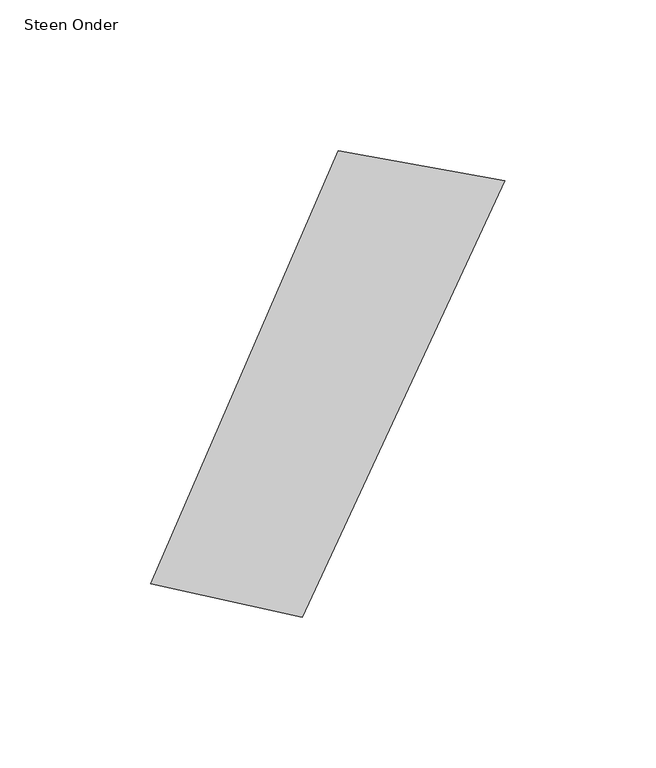
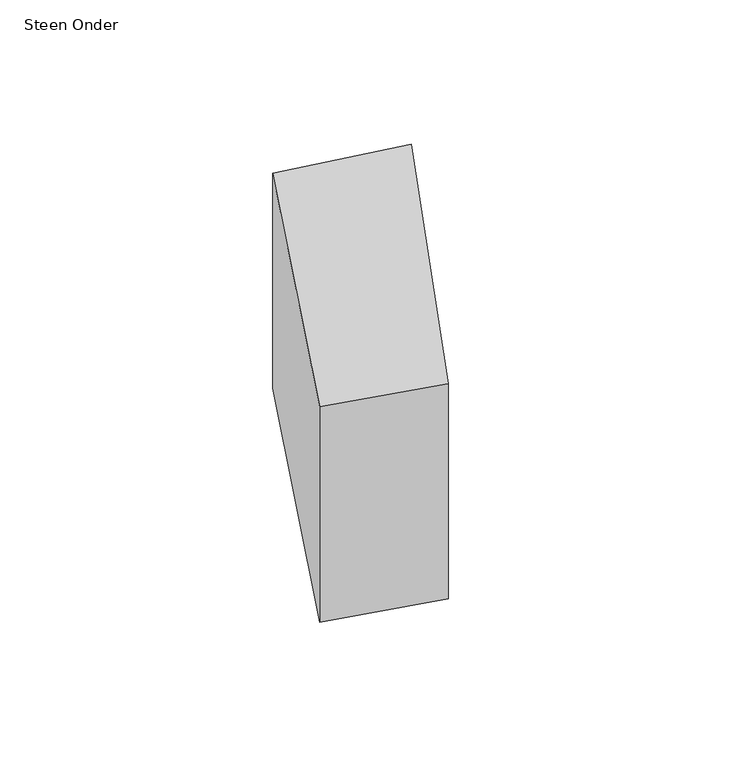
"""IFC4 building model written with IfcOpenShell, lengths in millimetres: proxy geometry, 00_GMA_steen_versie_4 : Steen Onder."""

from ifc_helpers import new_model, si_unit, origin, origin_with_axes, place, context, project, spatial, polyline, outline, extrude, source, transform, mapped, element, save


def steen_onder_ea4eff59(model_context):
    return source(origin(), model_context, "Body", "SweptSolid", [
        extrude(outline(polyline([(133.1834869, 139.6210071), (66.0338965, -4.9121836), (15.9385421, 6.1101542), (77.9749462, 149.4742626), (133.1834869, 139.6210071)])), origin_with_axes(), (0.0, 0.0, 1.0), 100.0),
    ])


if __name__ == "__main__":
    model = new_model("IFC4")
    model_context = context("Model", 3, world=origin())
    ifc_project = project(units=[si_unit("LENGTHUNIT", "METRE", prefix="MILLI")], contexts=[model_context])
    site = spatial("IfcSite", under=ifc_project)
    building = spatial("IfcBuilding", under=site)
    placement = place(None, origin())
    steen_onder_shape = steen_onder_ea4eff59(model_context)
    element("IfcBuildingElementProxy", 1, Name="00_GMA_steen_versie_4 : Steen Onder", ObjectType="00_GMA_steen_versie_4 : Steen Onder", at=placement, inside=building, context=model_context, shape_type="MappedRepresentation", body=[
        mapped(steen_onder_shape, transform((0.0, 0.0, 0.0), x_axis=(1.0, 0.0, 0.0), y_axis=(0.0, 1.0, 0.0), z_axis=(0.0, 0.0, 1.0))),
    ])
    save(model, "model.ifc")

# Revit data of these elements
# Type "00_GMA_steen_versie_4 : Steen Onder"
#   StootVoegHalfBoven [instance default] = 5 mm
#   StootVoegHalf [instance default] = 5 mm
#   StootVoegBreedteOnder = 10 mm
#   StootVoegBreedteBoven = 10 mm
#   Steendikte = 100 mm
#   LintVoegOnderHalf = 0 mm
#   LintVoegOnder = 0 mm
#   LintVoegBovenHalf = 5 mm
#   LintVoegBoven = 10 mm
#   materiaal = none
#   MateriaalVoeg = none
#   Default Elevation = 0
